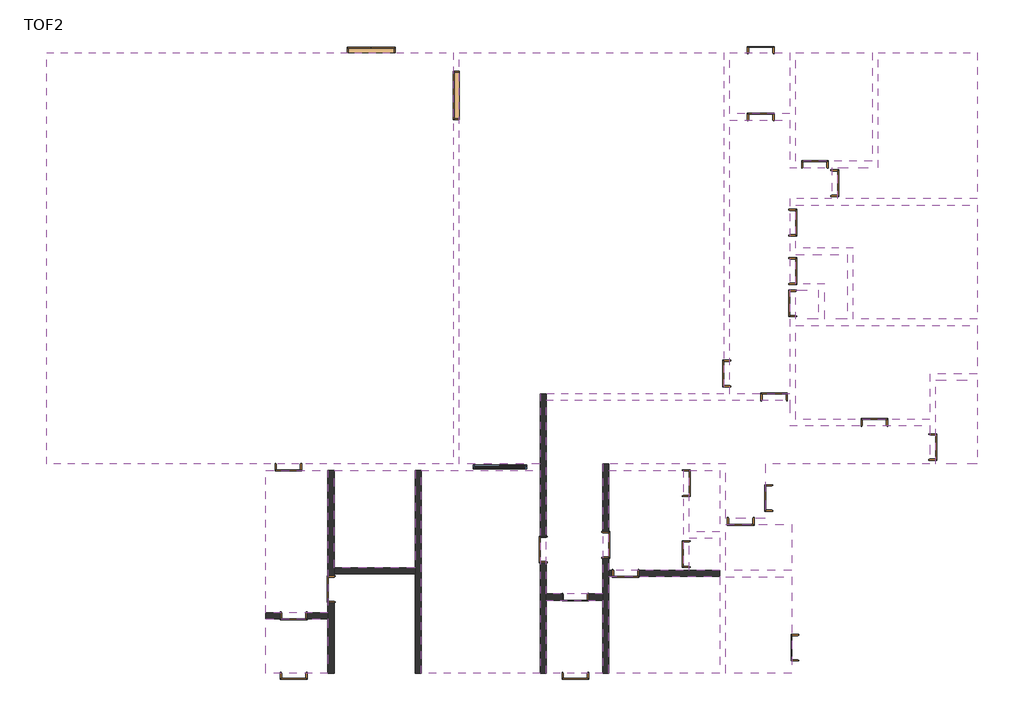
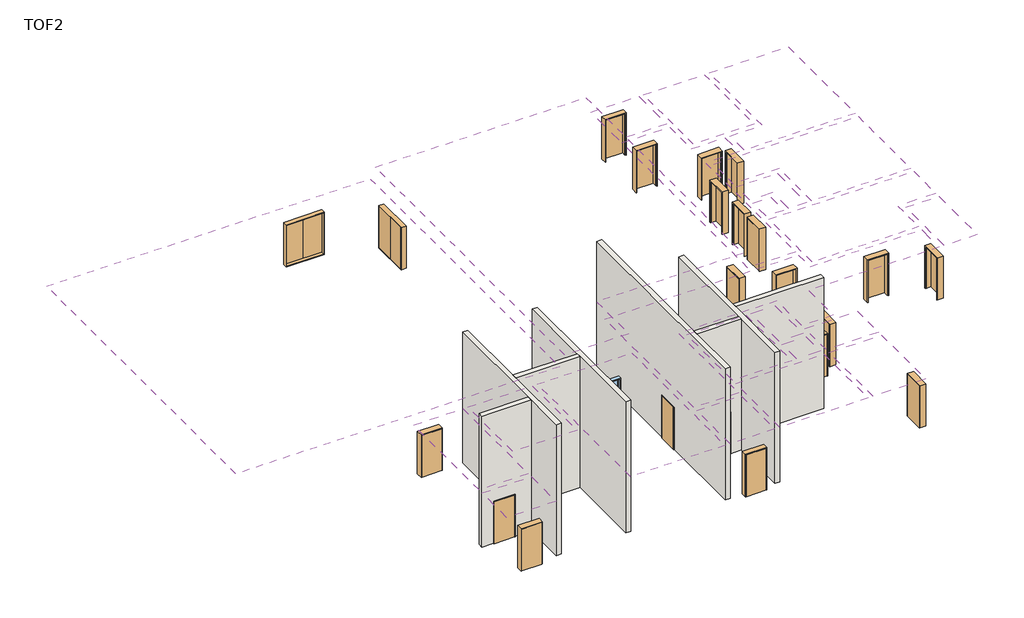
# One storey: 27 doors, 23 coverings, 8 walls, 1 window.
# Revit data of these elements (continued)
# Type "Sliding Window : H_WD_AR_B11_Sliding_Steel Window_DG_W2000xH1000" (continued)
#   Wall Closure = (empty or 0)
# Element 1 (IfcCovering, "H_CE_AR_B09_Acoustic Ceiling_T Bar_600x600x9T")
#   Height Offset From Level = 3000 mm
#   Phase Created = New Construction
# Element 2 (IfcCovering, "H_CE_AR_B09_Acoustic Ceiling_T Bar_600x600x9T")
#   Height Offset From Level = 3500 mm
#   Phase Created = New Construction
# Elements 3, 4, 5, 6, 7, 8, 9, 10, 11, 12, 13, 14, 15, 16, 17, 18, 19, 20, 21, 22, 23 (IfcCovering, "H_CE_AR_B09_Acoustic Ceiling_T Bar_600x600x9T")
#   Height Offset From Level = 2700 mm
#   Phase Created = New Construction
# Elements 24, 25 (IfcDoor, "Double Door_Steel : H_DR_AR_B12_Double Door_Steel_W2000xH2100")
#   H_Door Style Name = "Steel Door_Double"
#   H_Door_Frame = "Steel"
#   H_Door_Leaf = "Steel"
#   H_Door_Vision = "N.A"
#   H_Door_Panic = "N.A"
#   H_Door_Style Remark = ""
#   H_Door_Fire Rating = "NA/0.5/1.0\n/1.5/2.0"
#   H_Door Style No = DD11
#   Phase Created = New Construction
# Elements 26, 27, 28, 29, 30, 31, 32, 33, 34, 35, 36, 37, 38, 39, 40, 41, 42, 43, 44, 45, 46, 47, 48, 49, 50 (IfcDoor, "Single Door_Steel : H_DR_AR_B12_Single Door_Steel_W1000xH2100")
#   H_Door Style Name = "Steel Door_Single"
#   H_Door_Frame = "Steel"
#   H_Door_Leaf = "Steel"
#   H_Door_Vision = "N.A"
#   H_Door_Panic = "N.A"
#   H_Door_Style Remark = "Steel Door w/ Steel Frame"
#   H_Door_Fire Rating = "NA/0.5/1.0\n/1.5/2.0"
#   H_Door Style No = SD11
#   Phase Created = New Construction
# Elements 51, 52, 53, 54, 55, 56, 57, 58 (IfcWall, "H_WA_AR_B02_Int Wall_Block T200")
#   H_Wall Style Name = "Block Wall"
#   H_Wall-Base Material-1 = "Concrete Block"
#   H_Wall-Base Material-2 = ""
#   H_Wall_Finish-In = "Acrylic Emulsion Paint on Cement Plaster"
#   H_Wall_Base Material-3 = ""
#   H_Wall_Finish-Ex = "Acrylic Emulsion Paint on Cement Plaster"
#   H_Wall_Style Remark = "WM : Reinforced Concrete Block\n     50mm<THK≤100mm / 100mm<THK≤200mm / 200mm<THK"
#   Top Offset = 0 mm
#   Base Offset = 0 mm
#   wall height = 6500 mm
#   H_Wall Style No = IW21
#   Phase Created = New Construction
#   Base Constraint = TOF2
#   Top Constraint = TOC
#   Materials on its faces: "Default Wall"
# Element 59 (IfcWindow, "Sliding Window : H_WD_AR_B11_Sliding_Steel Window_DG_W2000xH1000")
#   Mark = "FRW-01"
#   H_Window Style Name = "Steel Window_DG_Comb"
#   H_Window_Glass = "Double Glazing"
#   H_Window_Frame = "Steel"
#   H_Window_Fire Rating = "NA/0.5/1.0"
#   H_Window_Style Remark = ""
#   H_Window Style No = WN42
#   Phase Created = New Construction
# Materials
#   "Default Wall": class "Miscellaneous", colour RGB 80 80 80, transparency 0
# Room at (8960, 18159.521) mm, phase "New Construction", upper level "TOC", upper offset 2000 mm, lower offset -2000 mm
#   Comments = ""
#   Number = "101"
#   Name = "MECHANICAL ROOM"
#   H_Floor Finish Style Name = "Non-Slip Epoxy Paint"
#   H_Floor Base Material = "Concrete Slab / Steel Trowel Finish"
#   H_Wall-Base Material-1 = "Masonry Wall"
#   H_Skirt Finish Style Name = "Epoxy Paint"
#   H_Wall-Base Material-2 = ""
#   H_Wall-Base Material-3 = "Plastering"
#   H_Floor-Base Material-1 = "Concrete Slab"
#   H_Floor-Base Material-2 = "Steel Trowel Finish"
#   H_Floor-Base Material-3 = ""
#   H_Floor-Base Material-4 = ""
#   H_Floor-Base Material-5 = ""
#   H_Floor Finish-1 = "Epoxy Paint"
#   H_Floor Finish-2 = ""
#   H_Floor Finish Remark = "*WM 기준 확인 필요 Epoxy Paint \n(용제형, 0.1mm 이하) : epoxy resin + polyamine hardener(경화제)"
#   H_Skirt Base Material = "Same as Wall"
#   H_Skirt-Base Material-1 = ""
#   H_Skirt-Base Material-2 = ""
#   H_Skirt-Base Material-3 = ""
#   H_Skirt-Base Material-4 = ""
#   H_Skirt-Base Material-5 = ""
#   H_Skirt Finish-1 = "Epoxy Paint"
#   H_Skirt Finish-2 = ""
#   H_Skirt Finish Remark = "SACE"
#   H_Wall Finish Style Name = "Acrylic Emulsion Paint"
#   H_Wall Base Material = "Masonry Wall / Cement Plaster"
#   H_Wall-Base Material-4 = ""
#   H_Wall-Base Material-5 = ""
#   H_Wall Finish-1 = "Acrylic Emulsion Paint"
#   H_Wall Finish-2 = ""
#   H_Wall Finish Remark = "T13 Plaster"
#   H_Ceiling Finish Style Name = "Acrylic Emulsion Paint"
#   H_Ceiling Base Material = "Concrete Slab / Fair Faced Concrete"
#   H_Ceiling-Base Material-1 = "(Concrete Slab)"
#   H_Ceiling-Base Material-2 = ""
#   H_Ceiling-Base Material-3 = ""
#   H_Ceiling-Base Material-4 = ""
#   H_Ceiling-Base Material-5 = ""
#   H_Ceiling Finish-1 = "Acrylic Emulsion Paint"
#   H_Ceiling Finish-2 = ""
#   H_Ceiling Finish Remark = "SACE"
#   Floor Finish Style No = F06A
#   Skirt Finish Style No = B03
#   Wall Finish Style No = W01B
#   Ceiling Finish Style No = C01
# Room at (8960, 6314.521) mm, phase "New Construction", upper level "TOC", upper offset 2000 mm, lower offset -2000 mm
#   Comments = ""
#   Number = "112"
#   Name = "ELECTRICAL ROOM(SS08)"
#   H_Floor Finish Style Name = "Non-Slip Epoxy Paint"
#   H_Floor Base Material = "Concrete Slab / Screed"
#   H_Wall-Base Material-1 = "Masonry Wall"
#   H_Skirt Finish Style Name = "Epoxy Paint"
#   H_Wall-Base Material-2 = ""
#   H_Wall-Base Material-3 = "Plastering"
#   H_Floor-Base Material-1 = "Concrete Slab"
#   H_Floor-Base Material-2 = ""
#   H_Floor-Base Material-3 = "Screed"
#   H_Floor-Base Material-4 = ""
#   H_Floor-Base Material-5 = ""
#   H_Floor Finish-1 = "Epoxy Paint"
#   H_Floor Finish-2 = ""
#   H_Floor Finish Remark = "*WM 기준 확인 필요 Epoxy Paint \n(용제형, 0.1mm 이하) : epoxy resin + polyamine hardener(경화제)"
#   H_Skirt Base Material = "Same as Wall"
#   H_Skirt-Base Material-1 = ""
#   H_Skirt-Base Material-2 = ""
#   H_Skirt-Base Material-3 = ""
#   H_Skirt-Base Material-4 = ""
#   H_Skirt-Base Material-5 = ""
#   H_Skirt Finish-1 = "Epoxy Paint"
#   H_Skirt Finish-2 = ""
#   H_Skirt Finish Remark = "SACE"
#   H_Wall Finish Style Name = "Acrylic Emulsion Paint"
#   H_Wall Base Material = "Masonry Wall / Cement Plaster"
#   H_Wall-Base Material-4 = ""
#   H_Wall-Base Material-5 = ""
#   H_Wall Finish-1 = "Acrylic Emulsion Paint"
#   H_Wall Finish-2 = ""
#   H_Wall Finish Remark = "T13 Plaster"
#   H_Ceiling Finish Style Name = "Acrylic Emulsion Paint"
#   H_Ceiling Base Material = "Concrete Slab / Fair Faced Concrete"
#   H_Ceiling-Base Material-1 = "(Concrete Slab)"
#   H_Ceiling-Base Material-2 = ""
#   H_Ceiling-Base Material-3 = ""
#   H_Ceiling-Base Material-4 = ""
#   H_Ceiling-Base Material-5 = ""
#   H_Ceiling Finish-1 = "Acrylic Emulsion Paint"
#   H_Ceiling Finish-2 = ""
#   H_Ceiling Finish Remark = "SACE"
#   Floor Finish Style No = F06B
#   Skirt Finish Style No = B03
#   Wall Finish Style No = W01B
#   Ceiling Finish Style No = C01
# Room at (25745, 16214.521) mm, phase "New Construction", upper level "TOC", upper offset 2000 mm, lower offset -2000 mm
#   Comments = ""
#   Number = "102"
#   Name = "RACK ROOM"
#   H_Floor Finish Style Name = "Anti-Dust Epoxy Paint / Anti-Static Vinyl Tile on Raised Floor"
#   H_Floor Base Material = "Concrete Slab / Steel Trowel Finish"
#   H_Wall-Base Material-1 = "Masonry Wall"
#   H_Skirt Finish Style Name = "Coved Vinyl Tile"
#   H_Wall-Base Material-2 = ""
#   H_Wall-Base Material-3 = "Plastering"
#   H_Floor-Base Material-1 = "Concrete Slab"
#   H_Floor-Base Material-2 = "Steel Trowel Finish"
#   H_Floor-Base Material-3 = ""
#   H_Floor-Base Material-4 = ""
#   H_Floor-Base Material-5 = "Raised Floor_Anti-Static Vinyl Tile"
#   H_Floor Finish-1 = "Anti-Dust Paint"
#   H_Floor Finish-2 = "Raised Floor_Anti-Static Vinyl Tile"
#   H_Floor Finish Remark = "600x600, H=1000"
#   H_Skirt Base Material = "Same as Wall"
#   H_Skirt-Base Material-1 = ""
#   H_Skirt-Base Material-2 = ""
#   H_Skirt-Base Material-3 = ""
#   H_Skirt-Base Material-4 = ""
#   H_Skirt-Base Material-5 = ""
#   H_Skirt Finish-1 = "Vinyl Tile"
#   H_Skirt Finish-2 = ""
#   H_Skirt Finish Remark = "Vinyl Tile = PVC Tile (polyvinyl chloride)"
#   H_Wall Finish Style Name = "Acrylic Emulsion Paint"
#   H_Wall Base Material = "Masonry Wall / Cement Plaster"
#   H_Wall-Base Material-4 = ""
#   H_Wall-Base Material-5 = ""
#   H_Wall Finish-1 = "Acrylic Emulsion Paint"
#   H_Wall Finish-2 = ""
#   H_Wall Finish Remark = "T13 Plaster"
#   H_Ceiling Finish Style Name = "Suspended Acoustic Tiled Ceiling (M-Bar)"
#   H_Ceiling Base Material = "Concrete Slab / Fair Faced Concrete"
#   H_Ceiling-Base Material-1 = "(Concrete Slab)"
#   H_Ceiling-Base Material-2 = "(Fair Faced Concrete)"
#   H_Ceiling-Base Material-3 = ""
#   H_Ceiling-Base Material-4 = ""
#   H_Ceiling-Base Material-5 = "Acoustic Tiled Ceiling System (M-Bar)"
#   H_Ceiling Finish-1 = "Acoustic Tiled Ceiling System (M-Bar)"
#   H_Ceiling Finish-2 = ""
#   H_Ceiling Finish Remark = ""
#   Floor Finish Style No = F91
#   Skirt Finish Style No = B35
#   Wall Finish Style No = W01B
#   Ceiling Finish Style No = C95A
# Room at (22095, 4359.521) mm, phase "New Construction", upper level "TOC", upper offset 2000 mm, lower offset -2000 mm
#   Comments = ""
#   Number = "114"
#   Name = "BATTERY ROOM"
#   H_Floor Finish Style Name = "Acid Resistant Ceramic Tile"
#   H_Floor Base Material = "Concrete Slab / Steel Trowel Finish"
#   H_Wall-Base Material-1 = "Masonry Wall"
#   H_Skirt Finish Style Name = "Coved Vinyl Tile"
#   H_Wall-Base Material-2 = ""
#   H_Wall-Base Material-3 = "Plastering"
#   H_Floor-Base Material-1 = "Concrete Slab"
#   H_Floor-Base Material-2 = "Steel Trowel Finish"
#   H_Floor-Base Material-3 = ""
#   H_Floor-Base Material-4 = ""
#   H_Floor-Base Material-5 = "Acid/Alkaline Resistant Tile"
#   H_Floor Finish-1 = "Acid/Alkaline Resistant Tile"
#   H_Floor Finish-2 = ""
#   H_Floor Finish Remark = "*WM : Bonding용 Mortar은 Tile에 포함\n*Slope 용 Screed만 별도 구분 (Concrete 바닥 단차 발생하는 경우 Only)"
#   H_Skirt Base Material = "Same as Wall"
#   H_Skirt-Base Material-1 = ""
#   H_Skirt-Base Material-2 = ""
#   H_Skirt-Base Material-3 = ""
#   H_Skirt-Base Material-4 = ""
#   H_Skirt-Base Material-5 = ""
#   H_Skirt Finish-1 = "Vinyl Tile"
#   H_Skirt Finish-2 = ""
#   H_Skirt Finish Remark = "Vinyl Tile = PVC Tile (polyvinyl chloride)"
#   H_Wall Finish Style Name = "Acid Resistant Paint"
#   H_Wall Base Material = "Masonry Wall / Cement Plaster"
#   H_Wall-Base Material-4 = ""
#   H_Wall-Base Material-5 = ""
#   H_Wall Finish-1 = "Acid/Alkaline Resistant Paint"
#   H_Wall Finish-2 = ""
#   H_Wall Finish Remark = "T13 Plaster"
#   H_Ceiling Finish Style Name = "Acrylic Emulsion Paint"
#   H_Ceiling Base Material = "Concrete Slab / Fair Faced Concrete"
#   H_Ceiling-Base Material-1 = "(Concrete Slab)"
#   H_Ceiling-Base Material-2 = ""
#   H_Ceiling-Base Material-3 = ""
#   H_Ceiling-Base Material-4 = ""
#   H_Ceiling-Base Material-5 = ""
#   H_Ceiling Finish-1 = "Acrylic Emulsion Paint"
#   H_Ceiling Finish-2 = ""
#   H_Ceiling Finish Remark = "SACE"
#   Floor Finish Style No = F32A
#   Skirt Finish Style No = B35
#   Wall Finish Style No = W04B
#   Ceiling Finish Style No = C01
# Room at (34300, 4359.521) mm, phase "New Construction", upper level "TOC", upper offset 2000 mm, lower offset -2000 mm
#   Comments = ""
#   Number = "118"
#   Name = "DRIVERS LOUNGE"
#   H_Floor Finish Style Name = "Vinyl Tile"
#   H_Floor Base Material = "Concrete Slab / Steel Trowel Finish"
#   H_Wall-Base Material-1 = "Masonry Wall"
#   H_Skirt Finish Style Name = "Coved Vinyl Tile"
#   H_Wall-Base Material-2 = ""
#   H_Wall-Base Material-3 = "Plastering"
#   H_Floor-Base Material-1 = "Concrete Slab"
#   H_Floor-Base Material-2 = "Steel Trowel Finish"
#   H_Floor-Base Material-3 = ""
#   H_Floor-Base Material-4 = ""
#   H_Floor-Base Material-5 = "Vinyl Tile"
#   H_Floor Finish-1 = "Vinyl Tile"
#   H_Floor Finish-2 = ""
#   H_Floor Finish Remark = ""
#   H_Skirt Base Material = "Same as Wall"
#   H_Skirt-Base Material-1 = ""
#   H_Skirt-Base Material-2 = ""
#   H_Skirt-Base Material-3 = ""
#   H_Skirt-Base Material-4 = ""
#   H_Skirt-Base Material-5 = ""
#   H_Skirt Finish-1 = "Vinyl Tile"
#   H_Skirt Finish-2 = ""
#   H_Skirt Finish Remark = "Vinyl Tile = PVC Tile (polyvinyl chloride)"
#   H_Wall Finish Style Name = "Acrylic Emulsion Paint"
#   H_Wall Base Material = "Masonry Wall / Cement Plaster"
#   H_Wall-Base Material-4 = ""
#   H_Wall-Base Material-5 = ""
#   H_Wall Finish-1 = "Acrylic Emulsion Paint"
#   H_Wall Finish-2 = ""
#   H_Wall Finish Remark = "T13 Plaster"
#   H_Ceiling Finish Style Name = "Suspended Acoustic Tiled Ceiling (M-Bar)"
#   H_Ceiling Base Material = "Concrete Slab / Fair Faced Concrete"
#   H_Ceiling-Base Material-1 = "(Concrete Slab)"
#   H_Ceiling-Base Material-2 = "(Fair Faced Concrete)"
#   H_Ceiling-Base Material-3 = ""
#   H_Ceiling-Base Material-4 = ""
#   H_Ceiling-Base Material-5 = "Acoustic Tiled Ceiling System (M-Bar)"
#   H_Ceiling Finish-1 = "Acoustic Tiled Ceiling System (M-Bar)"
#   H_Ceiling Finish-2 = ""
#   H_Ceiling Finish Remark = ""
#   Floor Finish Style No = F34A
#   Skirt Finish Style No = B35
#   Wall Finish Style No = W01B
#   Ceiling Finish Style No = C95A
# Room at (38475, 15984.521) mm, phase "New Construction", upper level "TOC", upper offset 2000 mm, lower offset -2000 mm
#   Comments = ""
#   Number = "103"
#   Name = "CONTROL ROOM"
#   H_Floor Finish Style Name = "Anti-Dust Epoxy Paint / Anti-Static Vinyl Tile on Raised Floor"
#   H_Floor Base Material = "Concrete Slab / Steel Trowel Finish"
#   H_Wall-Base Material-1 = "Masonry Wall"
#   H_Skirt Finish Style Name = "Coved Vinyl Tile"
#   H_Wall-Base Material-2 = ""
#   H_Wall-Base Material-3 = "Plastering"
#   H_Floor-Base Material-1 = "Concrete Slab"
#   H_Floor-Base Material-2 = "Steel Trowel Finish"
#   H_Floor-Base Material-3 = ""
#   H_Floor-Base Material-4 = ""
#   H_Floor-Base Material-5 = "Raised Floor_Anti-Static Vinyl Tile"
#   H_Floor Finish-1 = "Anti-Dust Paint"
#   H_Floor Finish-2 = "Raised Floor_Anti-Static Vinyl Tile"
#   H_Floor Finish Remark = "600x600, H=1000"
#   H_Skirt Base Material = "Same as Wall"
#   H_Skirt-Base Material-1 = ""
#   H_Skirt-Base Material-2 = ""
#   H_Skirt-Base Material-3 = ""
#   H_Skirt-Base Material-4 = ""
#   H_Skirt-Base Material-5 = ""
#   H_Skirt Finish-1 = "Vinyl Tile"
#   H_Skirt Finish-2 = ""
#   H_Skirt Finish Remark = "Vinyl Tile = PVC Tile (polyvinyl chloride)"
#   H_Wall Finish Style Name = "Acrylic Emulsion Paint"
#   H_Wall Base Material = "Masonry Wall / Cement Plaster"
#   H_Wall-Base Material-4 = ""
#   H_Wall-Base Material-5 = ""
#   H_Wall Finish-1 = "Acrylic Emulsion Paint"
#   H_Wall Finish-2 = ""
#   H_Wall Finish Remark = "T13 Plaster"
#   H_Ceiling Finish Style Name = "Suspended Acoustic Tiled Ceiling (M-Bar)"
#   H_Ceiling Base Material = "Concrete Slab / Fair Faced Concrete"
#   H_Ceiling-Base Material-1 = "(Concrete Slab)"
#   H_Ceiling-Base Material-2 = "(Fair Faced Concrete)"
#   H_Ceiling-Base Material-3 = ""
#   H_Ceiling-Base Material-4 = ""
#   H_Ceiling-Base Material-5 = "Acoustic Tiled Ceiling System (M-Bar)"
#   H_Ceiling Finish-1 = "Acoustic Tiled Ceiling System (M-Bar)"
#   H_Ceiling Finish-2 = ""
#   H_Ceiling Finish Remark = ""
#   Floor Finish Style No = F91
#   Skirt Finish Style No = B35
#   Wall Finish Style No = W01B
#   Ceiling Finish Style No = C95A
# Room at (41230, 2411.673) mm, phase "New Construction", upper level "TOC", upper offset 2000 mm, lower offset -2000 mm
#   Comments = ""
#   Number = "122"
#   Name = "TOILETS"
#   H_Floor Finish Style Name = "Non-Slip Unglazed Ceramic Tile"
#   H_Floor Base Material = "Concrete Slab / Screed / Liquid Waterproofing"
#   H_Wall-Base Material-1 = "Masonry Wall"
#   H_Skirt Finish Style Name = "Coved Ceramic Tile"
#   H_Wall-Base Material-2 = ""
#   H_Wall-Base Material-3 = ""
#   H_Floor-Base Material-1 = "Concrete Slab"
#   H_Floor-Base Material-2 = ""
#   H_Floor-Base Material-3 = "Screed"
#   H_Floor-Base Material-4 = "Liquid Waterproofing"
#   H_Floor-Base Material-5 = "Ceramic Tile"
#   H_Floor Finish-1 = "Ceramic Tile"
#   H_Floor Finish-2 = ""
#   H_Floor Finish Remark = ""
#   H_Skirt Base Material = "Same as Wall"
#   H_Skirt-Base Material-1 = ""
#   H_Skirt-Base Material-2 = ""
#   H_Skirt-Base Material-3 = ""
#   H_Skirt-Base Material-4 = ""
#   H_Skirt-Base Material-5 = ""
#   H_Skirt Finish-1 = "Glazed Ceramic Tile"
#   H_Skirt Finish-2 = ""
#   H_Skirt Finish Remark = ""
#   H_Wall Finish Style Name = "Glazed Ceramic Tile (≤C.H+100) / No Paint (>C.H+100)"
#   H_Wall Base Material = "Masonry Wall / Liquid Waterproofing"
#   H_Wall-Base Material-4 = "Liquid Waterproofing"
#   H_Wall-Base Material-5 = "Glazed Ceramic Tile"
#   H_Wall Finish-1 = "Glazed Ceramic Tile"
#   H_Wall Finish-2 = ""
#   H_Wall Finish Remark = "Below Suspended Ceiling\nGlazed Ceramic Tile(≤C.H+100) + Liquid Waterproofing / No Paint (>C.H+100)"
#   H_Ceiling Finish Style Name = "Suspended Moisture Resistant Tiled Ceiling (M-Bar)"
#   H_Ceiling Base Material = "Concrete Slab / Fair Faced Concrete"
#   H_Ceiling-Base Material-1 = "(Concrete Slab)"
#   H_Ceiling-Base Material-2 = "(Fair Faced Concrete)"
#   H_Ceiling-Base Material-3 = ""
#   H_Ceiling-Base Material-4 = ""
#   H_Ceiling-Base Material-5 = "Moisture Resistant Tiled Ceiling System (M-Bar)"
#   H_Ceiling Finish-1 = "Moisture Resistant Tiled Ceiling System (M-Bar)"
#   H_Ceiling Finish-2 = ""
#   H_Ceiling Finish Remark = ""
#   Floor Finish Style No = F31B
#   Skirt Finish Style No = B32
#   Wall Finish Style No = W32B
#   Ceiling Finish Style No = C96A
# Room at (49122.5, 4434.521) mm, phase "New Construction", upper level "TOC", upper offset 2000 mm, lower offset -2000 mm
#   Comments = ""
#   Number = "125"
#   Name = "MAINTENANCE WORKSHOP"
#   H_Floor Finish Style Name = "Non-Slip Epoxy Paint"
#   H_Floor Base Material = "Concrete Slab / Steel Trowel Finish"
#   H_Wall-Base Material-1 = "Masonry Wall"
#   H_Skirt Finish Style Name = "Epoxy Paint"
#   H_Wall-Base Material-2 = ""
#   H_Wall-Base Material-3 = "Plastering"
#   H_Floor-Base Material-1 = "Concrete Slab"
#   H_Floor-Base Material-2 = "Steel Trowel Finish"
#   H_Floor-Base Material-3 = ""
#   H_Floor-Base Material-4 = ""
#   H_Floor-Base Material-5 = ""
#   H_Floor Finish-1 = "Epoxy Paint"
#   H_Floor Finish-2 = ""
#   H_Floor Finish Remark = "*WM 기준 확인 필요 Epoxy Paint \n(용제형, 0.1mm 이하) : epoxy resin + polyamine hardener(경화제)"
#   H_Skirt Base Material = "Same as Wall"
#   H_Skirt-Base Material-1 = ""
#   H_Skirt-Base Material-2 = ""
#   H_Skirt-Base Material-3 = ""
#   H_Skirt-Base Material-4 = ""
#   H_Skirt-Base Material-5 = ""
#   H_Skirt Finish-1 = "Epoxy Paint"
#   H_Skirt Finish-2 = ""
#   H_Skirt Finish Remark = "SACE"
#   H_Wall Finish Style Name = "Acrylic Emulsion Paint"
#   H_Wall Base Material = "Masonry Wall / Cement Plaster"
#   H_Wall-Base Material-4 = ""
#   H_Wall-Base Material-5 = ""
#   H_Wall Finish-1 = "Acrylic Emulsion Paint"
#   H_Wall Finish-2 = ""
#   H_Wall Finish Remark = "T13 Plaster"
#   H_Ceiling Finish Style Name = "Acrylic Emulsion Paint"
#   H_Ceiling Base Material = "Concrete Slab / Fair Faced Concrete"
#   H_Ceiling-Base Material-1 = "(Concrete Slab)"
#   H_Ceiling-Base Material-2 = ""
#   H_Ceiling-Base Material-3 = ""
#   H_Ceiling-Base Material-4 = ""
#   H_Ceiling-Base Material-5 = ""
#   H_Ceiling Finish-1 = "Acrylic Emulsion Paint"
#   H_Ceiling Finish-2 = ""
#   H_Ceiling Finish Remark = "SACE"
#   Floor Finish Style No = F06A
#   Skirt Finish Style No = B03
#   Wall Finish Style No = W01B
#   Ceiling Finish Style No = C01
# Room at (40475, 6276.673) mm, phase "New Construction", upper level "TOC", upper offset 2000 mm, lower offset -2000 mm
#   Comments = ""
#   Number = "121"
#   Name = "LOCKER"
#   H_Floor Finish Style Name = "Non-Slip Unglazed Ceramic Tile"
#   H_Floor Base Material = "Concrete Slab / Steel Trowel Finish"
#   H_Wall-Base Material-1 = "Masonry Wall"
#   H_Skirt Finish Style Name = "Coved Ceramic Tile"
#   H_Wall-Base Material-2 = ""
#   H_Wall-Base Material-3 = ""
#   H_Floor-Base Material-1 = "Concrete Slab"
#   H_Floor-Base Material-2 = "Steel Trowel Finish"
#   H_Floor-Base Material-3 = ""
#   H_Floor-Base Material-4 = ""
#   H_Floor-Base Material-5 = "Ceramic Tile"
#   H_Floor Finish-1 = "Ceramic Tile"
#   H_Floor Finish-2 = ""
#   H_Floor Finish Remark = "*WM : Bonding용 Mortar은 Tile에 포함\n*Slope 용 Screed만 별도 구분 (Concrete 바닥 단차 발생하는 경우 Only)"
#   H_Skirt Base Material = "Same as Wall"
#   H_Skirt-Base Material-1 = ""
#   H_Skirt-Base Material-2 = ""
#   H_Skirt-Base Material-3 = ""
#   H_Skirt-Base Material-4 = ""
#   H_Skirt-Base Material-5 = ""
#   H_Skirt Finish-1 = "Glazed Ceramic Tile"
#   H_Skirt Finish-2 = ""
#   H_Skirt Finish Remark = ""
#   H_Wall Finish Style Name = "Glazed Ceramic Tile (≤C.H+100) / No Paint (>C.H+100)"
#   H_Wall Base Material = "Masonry Wall / Liquid Waterproofing"
#   H_Wall-Base Material-4 = "Liquid Waterproofing"
#   H_Wall-Base Material-5 = "Glazed Ceramic Tile"
#   H_Wall Finish-1 = "Glazed Ceramic Tile"
#   H_Wall Finish-2 = ""
#   H_Wall Finish Remark = "Below Suspended Ceiling\nGlazed Ceramic Tile(≤C.H+100) + Liquid Waterproofing / No Paint (>C.H+100)"
#   H_Ceiling Finish Style Name = "Suspended Moisture Resistant Tiled Ceiling (M-Bar)"
#   H_Ceiling Base Material = "Concrete Slab / Fair Faced Concrete"
#   H_Ceiling-Base Material-1 = "(Concrete Slab)"
#   H_Ceiling-Base Material-2 = "(Fair Faced Concrete)"
#   H_Ceiling-Base Material-3 = ""
#   H_Ceiling-Base Material-4 = ""
#   H_Ceiling-Base Material-5 = "Moisture Resistant Tiled Ceiling System (M-Bar)"
#   H_Ceiling Finish-1 = "Moisture Resistant Tiled Ceiling System (M-Bar)"
#   H_Ceiling Finish-2 = ""
#   H_Ceiling Finish Remark = ""
#   Floor Finish Style No = F31A
#   Skirt Finish Style No = B32
#   Wall Finish Style No = W32B
#   Ceiling Finish Style No = C96A
# Room at (42700, 7069.521) mm, phase "New Construction", upper level "TOC", upper offset 2000 mm, lower offset -2000 mm
#   Comments = ""
#   Number = "127"
#   Name = "SHOWER ROOM"
#   H_Floor Finish Style Name = "Non-Slip Unglazed Ceramic Tile"
#   H_Floor Base Material = "Concrete Slab / Screed / Liquid Waterproofing"
#   H_Wall-Base Material-1 = "Concrete Wall"
#   H_Skirt Finish Style Name = "Epoxy Paint"
#   H_Wall-Base Material-2 = ""
#   H_Wall-Base Material-3 = ""
#   H_Floor-Base Material-1 = "Concrete Slab"
#   H_Floor-Base Material-2 = ""
#   H_Floor-Base Material-3 = "Screed"
#   H_Floor-Base Material-4 = "Liquid Waterproofing"
#   H_Floor-Base Material-5 = "Ceramic Tile"
#   H_Floor Finish-1 = "Ceramic Tile"
#   H_Floor Finish-2 = ""
#   H_Floor Finish Remark = ""
#   H_Skirt Base Material = "Same as Wall"
#   H_Skirt-Base Material-1 = ""
#   H_Skirt-Base Material-2 = ""
#   H_Skirt-Base Material-3 = ""
#   H_Skirt-Base Material-4 = ""
#   H_Skirt-Base Material-5 = ""
#   H_Skirt Finish-1 = "Epoxy Paint"
#   H_Skirt Finish-2 = ""
#   H_Skirt Finish Remark = "SACE"
#   H_Wall Finish Style Name = "Glazed Ceramic Tile (≤C.H+100) / No Paint (>C.H+100)"
#   H_Wall Base Material = "Concrete Wall"
#   H_Wall-Base Material-4 = "No Waterproofing"
#   H_Wall-Base Material-5 = "Glazed Ceramic Tile"
#   H_Wall Finish-1 = "Glazed Ceramic Tile"
#   H_Wall Finish-2 = ""
#   H_Wall Finish Remark = "Below Suspended Ceiling\nGlazed Ceramic Tile(≤C.H+100) / No Paint (>C.H+100)"
#   H_Ceiling Finish Style Name = "Suspended Moisture Resistant Tiled Ceiling (M-Bar)"
#   H_Ceiling Base Material = "Concrete Slab / Fair Faced Concrete"
#   H_Ceiling-Base Material-1 = "(Concrete Slab)"
#   H_Ceiling-Base Material-2 = "(Fair Faced Concrete)"
#   H_Ceiling-Base Material-3 = ""
#   H_Ceiling-Base Material-4 = ""
#   H_Ceiling-Base Material-5 = "Moisture Resistant Tiled Ceiling System (M-Bar)"
#   H_Ceiling Finish-1 = "Moisture Resistant Tiled Ceiling System (M-Bar)"
#   H_Ceiling Finish-2 = ""
#   H_Ceiling Finish Remark = ""
#   Floor Finish Style No = F31B
#   Skirt Finish Style No = B03
#   Wall Finish Style No = W32C
#   Ceiling Finish Style No = C96A
# Room at (42700, 5046.673) mm, phase "New Construction", upper level "TOC", upper offset 2000 mm, lower offset -2000 mm
#   Comments = ""
#   Number = "128"
#   Name = "EWH ROOM"
#   H_Floor Finish Style Name = "Non-Slip Unglazed Ceramic Tile"
#   H_Floor Base Material = "Concrete Slab / Steel Trowel Finish"
#   H_Wall-Base Material-1 = "Masonry Wall"
#   H_Skirt Finish Style Name = "Epoxy Paint"
#   H_Wall-Base Material-2 = ""
#   H_Wall-Base Material-3 = "Plastering"
#   H_Floor-Base Material-1 = "Concrete Slab"
#   H_Floor-Base Material-2 = "Steel Trowel Finish"
#   H_Floor-Base Material-3 = ""
#   H_Floor-Base Material-4 = ""
#   H_Floor-Base Material-5 = "Ceramic Tile"
#   H_Floor Finish-1 = "Ceramic Tile"
#   H_Floor Finish-2 = ""
#   H_Floor Finish Remark = "*WM : Bonding용 Mortar은 Tile에 포함\n*Slope 용 Screed만 별도 구분 (Concrete 바닥 단차 발생하는 경우 Only)"
#   H_Skirt Base Material = "Same as Wall"
#   H_Skirt-Base Material-1 = ""
#   H_Skirt-Base Material-2 = ""
#   H_Skirt-Base Material-3 = ""
#   H_Skirt-Base Material-4 = ""
#   H_Skirt-Base Material-5 = ""
#   H_Skirt Finish-1 = "Epoxy Paint"
#   H_Skirt Finish-2 = ""
#   H_Skirt Finish Remark = "SACE"
#   H_Wall Finish Style Name = "Acrylic Emulsion Paint"
#   H_Wall Base Material = "Masonry Wall / Cement Plaster"
#   H_Wall-Base Material-4 = ""
#   H_Wall-Base Material-5 = ""
#   H_Wall Finish-1 = "Acrylic Emulsion Paint"
#   H_Wall Finish-2 = ""
#   H_Wall Finish Remark = "T13 Plaster"
#   H_Ceiling Finish Style Name = "Suspended Acoustic Tiled Ceiling (M-Bar)"
#   H_Ceiling Base Material = "Concrete Slab / Fair Faced Concrete"
#   H_Ceiling-Base Material-1 = "(Concrete Slab)"
#   H_Ceiling-Base Material-2 = "(Fair Faced Concrete)"
#   H_Ceiling-Base Material-3 = ""
#   H_Ceiling-Base Material-4 = ""
#   H_Ceiling-Base Material-5 = "Acoustic Tiled Ceiling System (M-Bar)"
#   H_Ceiling Finish-1 = "Acoustic Tiled Ceiling System (M-Bar)"
#   H_Ceiling Finish-2 = ""
#   H_Ceiling Finish Remark = ""
#   Floor Finish Style No = F31A
#   Skirt Finish Style No = B03
#   Wall Finish Style No = W01B
#   Ceiling Finish Style No = C95A
# Room at (52040, 9944.521) mm, phase "New Construction", upper level "TOC", upper offset 2000 mm, lower offset -2000 mm
#   Comments = ""
#   Number = "110"
#   Name = "ABLUTIONS"
#   H_Floor Finish Style Name = "Non-Slip Unglazed Ceramic Tile"
#   H_Floor Base Material = "Concrete Slab / Screed / Liquid Waterproofing"
#   H_Wall-Base Material-1 = "Masonry Wall"
#   H_Skirt Finish Style Name = "Coved Ceramic Tile"
#   H_Wall-Base Material-2 = ""
#   H_Wall-Base Material-3 = ""
#   H_Floor-Base Material-1 = "Concrete Slab"
#   H_Floor-Base Material-2 = ""
#   H_Floor-Base Material-3 = "Screed"
#   H_Floor-Base Material-4 = "Liquid Waterproofing"
#   H_Floor-Base Material-5 = "Ceramic Tile"
#   H_Floor Finish-1 = "Ceramic Tile"
#   H_Floor Finish-2 = ""
#   H_Floor Finish Remark = ""
#   H_Skirt Base Material = "Same as Wall"
#   H_Skirt-Base Material-1 = ""
#   H_Skirt-Base Material-2 = ""
#   H_Skirt-Base Material-3 = ""
#   H_Skirt-Base Material-4 = ""
#   H_Skirt-Base Material-5 = ""
#   H_Skirt Finish-1 = "Glazed Ceramic Tile"
#   H_Skirt Finish-2 = ""
#   H_Skirt Finish Remark = ""
#   H_Wall Finish Style Name = "Glazed Ceramic Tile (≤C.H+100) / No Paint (>C.H+100)"
#   H_Wall Base Material = "Masonry Wall / Liquid Waterproofing"
#   H_Wall-Base Material-4 = "Liquid Waterproofing"
#   H_Wall-Base Material-5 = "Glazed Ceramic Tile"
#   H_Wall Finish-1 = "Glazed Ceramic Tile"
#   H_Wall Finish-2 = ""
#   H_Wall Finish Remark = "Below Suspended Ceiling\nGlazed Ceramic Tile(≤C.H+100) + Liquid Waterproofing / No Paint (>C.H+100)"
#   H_Ceiling Finish Style Name = "Suspended Moisture Resistant Tiled Ceiling (M-Bar)"
#   H_Ceiling Base Material = "Concrete Slab / Fair Faced Concrete"
#   H_Ceiling-Base Material-1 = "(Concrete Slab)"
#   H_Ceiling-Base Material-2 = "(Fair Faced Concrete)"
#   H_Ceiling-Base Material-3 = ""
#   H_Ceiling-Base Material-4 = ""
#   H_Ceiling-Base Material-5 = "Moisture Resistant Tiled Ceiling System (M-Bar)"
#   H_Ceiling Finish-1 = "Moisture Resistant Tiled Ceiling System (M-Bar)"
#   H_Ceiling Finish-2 = ""
#   H_Ceiling Finish Remark = ""
#   Floor Finish Style No = F31B
#   Skirt Finish Style No = B32
#   Wall Finish Style No = W32B
#   Ceiling Finish Style No = C96A
# Room at (50360, 21134.521) mm, phase "New Construction", upper level "TOC", upper offset 2000 mm, lower offset -2000 mm
#   Comments = ""
#   Number = "106"
#   Name = "SHIFT SUPERVISOR/DAY SUPERVISOR"
#   H_Floor Finish Style Name = "Vinyl Tile"
#   H_Floor Base Material = "Concrete Slab / Steel Trowel Finish"
#   H_Wall-Base Material-1 = "Masonry Wall"
#   H_Skirt Finish Style Name = "Coved Vinyl Tile"
#   H_Wall-Base Material-2 = ""
#   H_Wall-Base Material-3 = "Plastering"
#   H_Floor-Base Material-1 = "Concrete Slab"
#   H_Floor-Base Material-2 = "Steel Trowel Finish"
#   H_Floor-Base Material-3 = ""
#   H_Floor-Base Material-4 = ""
#   H_Floor-Base Material-5 = "Vinyl Tile"
#   H_Floor Finish-1 = "Vinyl Tile"
#   H_Floor Finish-2 = ""
#   H_Floor Finish Remark = ""
#   H_Skirt Base Material = "Same as Wall"
#   H_Skirt-Base Material-1 = ""
#   H_Skirt-Base Material-2 = ""
#   H_Skirt-Base Material-3 = ""
#   H_Skirt-Base Material-4 = ""
#   H_Skirt-Base Material-5 = ""
#   H_Skirt Finish-1 = "Vinyl Tile"
#   H_Skirt Finish-2 = ""
#   H_Skirt Finish Remark = "Vinyl Tile = PVC Tile (polyvinyl chloride)"
#   H_Wall Finish Style Name = "Acrylic Emulsion Paint"
#   H_Wall Base Material = "Masonry Wall / Cement Plaster"
#   H_Wall-Base Material-4 = ""
#   H_Wall-Base Material-5 = ""
#   H_Wall Finish-1 = "Acrylic Emulsion Paint"
#   H_Wall Finish-2 = ""
#   H_Wall Finish Remark = "T13 Plaster"
#   H_Ceiling Finish Style Name = "Suspended Acoustic Tiled Ceiling (M-Bar)"
#   H_Ceiling Base Material = "Concrete Slab / Fair Faced Concrete"
#   H_Ceiling-Base Material-1 = "(Concrete Slab)"
#   H_Ceiling-Base Material-2 = "(Fair Faced Concrete)"
#   H_Ceiling-Base Material-3 = ""
#   H_Ceiling-Base Material-4 = ""
#   H_Ceiling-Base Material-5 = "Acoustic Tiled Ceiling System (M-Bar)"
#   H_Ceiling Finish-1 = "Acoustic Tiled Ceiling System (M-Bar)"
#   H_Ceiling Finish-2 = ""
#   H_Ceiling Finish Remark = ""
#   Floor Finish Style No = F34A
#   Skirt Finish Style No = B35
#   Wall Finish Style No = W01B
#   Ceiling Finish Style No = C95A
# Room at (44725, 22722.021) mm, phase "New Construction", upper level "TOC", upper offset 2000 mm, lower offset -2000 mm
#   Comments = ""
#   Number = "104"
#   Name = "AIR LOCK"
#   H_Floor Finish Style Name = "Vinyl Tile"
#   H_Floor Base Material = "Concrete Slab / Steel Trowel Finish"
#   H_Wall-Base Material-1 = "Masonry Wall"
#   H_Skirt Finish Style Name = "Coved Vinyl Tile"
#   H_Wall-Base Material-2 = ""
#   H_Wall-Base Material-3 = "Plastering"
#   H_Floor-Base Material-1 = "Concrete Slab"
#   H_Floor-Base Material-2 = "Steel Trowel Finish"
#   H_Floor-Base Material-3 = ""
#   H_Floor-Base Material-4 = ""
#   H_Floor-Base Material-5 = "Vinyl Tile"
#   H_Floor Finish-1 = "Vinyl Tile"
#   H_Floor Finish-2 = ""
#   H_Floor Finish Remark = ""
#   H_Skirt Base Material = "Same as Wall"
#   H_Skirt-Base Material-1 = ""
#   H_Skirt-Base Material-2 = ""
#   H_Skirt-Base Material-3 = ""
#   H_Skirt-Base Material-4 = ""
#   H_Skirt-Base Material-5 = ""
#   H_Skirt Finish-1 = "Vinyl Tile"
#   H_Skirt Finish-2 = ""
#   H_Skirt Finish Remark = "Vinyl Tile = PVC Tile (polyvinyl chloride)"
#   H_Wall Finish Style Name = "Acrylic Emulsion Paint"
#   H_Wall Base Material = "Masonry Wall / Cement Plaster"
#   H_Wall-Base Material-4 = ""
#   H_Wall-Base Material-5 = ""
#   H_Wall Finish-1 = "Acrylic Emulsion Paint"
#   H_Wall Finish-2 = ""
#   H_Wall Finish Remark = "T13 Plaster"
#   H_Ceiling Finish Style Name = "Suspended Acoustic Tiled Ceiling (M-Bar)"
#   H_Ceiling Base Material = "Concrete Slab / Fair Faced Concrete"
#   H_Ceiling-Base Material-1 = "(Concrete Slab)"
#   H_Ceiling-Base Material-2 = "(Fair Faced Concrete)"
#   H_Ceiling-Base Material-3 = ""
#   H_Ceiling-Base Material-4 = ""
#   H_Ceiling-Base Material-5 = "Acoustic Tiled Ceiling System (M-Bar)"
#   H_Ceiling Finish-1 = "Acoustic Tiled Ceiling System (M-Bar)"
#   H_Ceiling Finish-2 = ""
#   H_Ceiling Finish Remark = ""
#   Floor Finish Style No = F34A
#   Skirt Finish Style No = B35
#   Wall Finish Style No = W01B
#   Ceiling Finish Style No = C95A
# Room at (45470, 16157.021) mm, phase "New Construction", upper level "TOC", upper offset 2000 mm, lower offset -2000 mm
#   Comments = ""
#   Number = "107"
#   Name = "CORRIDOR"
#   H_Floor Finish Style Name = "Vinyl Tile"
#   H_Floor Base Material = "Concrete Slab / Steel Trowel Finish"
#   H_Wall-Base Material-1 = "Masonry Wall"
#   H_Skirt Finish Style Name = "Coved Vinyl Tile"
#   H_Wall-Base Material-2 = ""
#   H_Wall-Base Material-3 = "Plastering"
#   H_Floor-Base Material-1 = "Concrete Slab"
#   H_Floor-Base Material-2 = "Steel Trowel Finish"
#   H_Floor-Base Material-3 = ""
#   H_Floor-Base Material-4 = ""
#   H_Floor-Base Material-5 = "Vinyl Tile"
#   H_Floor Finish-1 = "Vinyl Tile"
#   H_Floor Finish-2 = ""
#   H_Floor Finish Remark = ""
#   H_Skirt Base Material = "Same as Wall"
#   H_Skirt-Base Material-1 = ""
#   H_Skirt-Base Material-2 = ""
#   H_Skirt-Base Material-3 = ""
#   H_Skirt-Base Material-4 = ""
#   H_Skirt-Base Material-5 = ""
#   H_Skirt Finish-1 = "Vinyl Tile"
#   H_Skirt Finish-2 = ""
#   H_Skirt Finish Remark = "Vinyl Tile = PVC Tile (polyvinyl chloride)"
#   H_Wall Finish Style Name = "Acrylic Emulsion Paint"
#   H_Wall Base Material = "Masonry Wall / Cement Plaster"
#   H_Wall-Base Material-4 = ""
#   H_Wall-Base Material-5 = ""
#   H_Wall Finish-1 = "Acrylic Emulsion Paint"
#   H_Wall Finish-2 = ""
#   H_Wall Finish Remark = "T13 Plaster"
#   H_Ceiling Finish Style Name = "Suspended Acoustic Tiled Ceiling (M-Bar)"
#   H_Ceiling Base Material = "Concrete Slab / Fair Faced Concrete"
#   H_Ceiling-Base Material-1 = "(Concrete Slab)"
#   H_Ceiling-Base Material-2 = "(Fair Faced Concrete)"
#   H_Ceiling-Base Material-3 = ""
#   H_Ceiling-Base Material-4 = ""
#   H_Ceiling-Base Material-5 = "Acoustic Tiled Ceiling System (M-Bar)"
#   H_Ceiling Finish-1 = "Acoustic Tiled Ceiling System (M-Bar)"
#   H_Ceiling Finish-2 = ""
#   H_Ceiling Finish Remark = ""
#   Floor Finish Style No = F34A
#   Skirt Finish Style No = B35
#   Wall Finish Style No = W01B
#   Ceiling Finish Style No = C95A
# Room at (47500, 21684.521) mm, phase "New Construction", upper level "TOC", upper offset 2000 mm, lower offset -2000 mm
#   Comments = ""
#   Number = "105"
#   Name = "LIBRARY"
#   H_Floor Finish Style Name = "Vinyl Tile"
#   H_Floor Base Material = "Concrete Slab / Steel Trowel Finish"
#   H_Wall-Base Material-1 = "Masonry Wall"
#   H_Skirt Finish Style Name = "Coved Vinyl Tile"
#   H_Wall-Base Material-2 = ""
#   H_Wall-Base Material-3 = "Plastering"
#   H_Floor-Base Material-1 = "Concrete Slab"
#   H_Floor-Base Material-2 = "Steel Trowel Finish"
#   H_Floor-Base Material-3 = ""
#   H_Floor-Base Material-4 = ""
#   H_Floor-Base Material-5 = "Vinyl Tile"
#   H_Floor Finish-1 = "Vinyl Tile"
#   H_Floor Finish-2 = ""
#   H_Floor Finish Remark = ""
#   H_Skirt Base Material = "Same as Wall"
#   H_Skirt-Base Material-1 = ""
#   H_Skirt-Base Material-2 = ""
#   H_Skirt-Base Material-3 = ""
#   H_Skirt-Base Material-4 = ""
#   H_Skirt-Base Material-5 = ""
#   H_Skirt Finish-1 = "Vinyl Tile"
#   H_Skirt Finish-2 = ""
#   H_Skirt Finish Remark = "Vinyl Tile = PVC Tile (polyvinyl chloride)"
#   H_Wall Finish Style Name = "Acrylic Emulsion Paint"
#   H_Wall Base Material = "Masonry Wall / Cement Plaster"
#   H_Wall-Base Material-4 = ""
#   H_Wall-Base Material-5 = ""
#   H_Wall Finish-1 = "Acrylic Emulsion Paint"
#   H_Wall Finish-2 = ""
#   H_Wall Finish Remark = "T13 Plaster"
#   H_Ceiling Finish Style Name = "Suspended Acoustic Tiled Ceiling (M-Bar)"
#   H_Ceiling Base Material = "Concrete Slab / Fair Faced Concrete"
#   H_Ceiling-Base Material-1 = "(Concrete Slab)"
#   H_Ceiling-Base Material-2 = "(Fair Faced Concrete)"
#   H_Ceiling-Base Material-3 = ""
#   H_Ceiling-Base Material-4 = ""
#   H_Ceiling-Base Material-5 = "Acoustic Tiled Ceiling System (M-Bar)"
#   H_Ceiling Finish-1 = "Acoustic Tiled Ceiling System (M-Bar)"
#   H_Ceiling Finish-2 = ""
#   H_Ceiling Finish Remark = ""
#   Floor Finish Style No = F34A
#   Skirt Finish Style No = B35
#   Wall Finish Style No = W01B
#   Ceiling Finish Style No = C95A
# Room at (49385, 11844.521) mm, phase "New Construction", upper level "TOC", upper offset 2000 mm, lower offset -2000 mm
#   Comments = ""
#   Number = "111"
#   Name = "PRAYER ROOM"
#   H_Floor Finish Style Name = "Carpet"
#   H_Floor Base Material = "(기존 Floor Finish)"
#   H_Wall-Base Material-1 = "Masonry Wall"
#   H_Skirt Finish Style Name = "Coved Vinyl Tile"
#   H_Wall-Base Material-2 = ""
#   H_Wall-Base Material-3 = "Plastering"
#   H_Floor-Base Material-1 = "Carpet"
#   H_Floor-Base Material-2 = ""
#   H_Floor-Base Material-3 = ""
#   H_Floor-Base Material-4 = ""
#   H_Floor-Base Material-5 = ""
#   H_Floor Finish-1 = ""
#   H_Floor Finish-2 = ""
#   H_Floor Finish Remark = "* 기존 Floor Finsh 위에 Mat 의 설치면적 만큼 별도의 Family 적용"
#   H_Skirt Base Material = "Same as Wall"
#   H_Skirt-Base Material-1 = ""
#   H_Skirt-Base Material-2 = ""
#   H_Skirt-Base Material-3 = ""
#   H_Skirt-Base Material-4 = ""
#   H_Skirt-Base Material-5 = ""
#   H_Skirt Finish-1 = "Vinyl Tile"
#   H_Skirt Finish-2 = ""
#   H_Skirt Finish Remark = "Vinyl Tile = PVC Tile (polyvinyl chloride)"
#   H_Wall Finish Style Name = "Acrylic Emulsion Paint"
#   H_Wall Base Material = "Masonry Wall / Cement Plaster"
#   H_Wall-Base Material-4 = ""
#   H_Wall-Base Material-5 = ""
#   H_Wall Finish-1 = "Acrylic Emulsion Paint"
#   H_Wall Finish-2 = ""
#   H_Wall Finish Remark = "T13 Plaster"
#   H_Ceiling Finish Style Name = "Suspended Acoustic Tiled Ceiling (M-Bar)"
#   H_Ceiling Base Material = "Concrete Slab / Fair Faced Concrete"
#   H_Ceiling-Base Material-1 = "(Concrete Slab)"
#   H_Ceiling-Base Material-2 = "(Fair Faced Concrete)"
#   H_Ceiling-Base Material-3 = ""
#   H_Ceiling-Base Material-4 = ""
#   H_Ceiling-Base Material-5 = "Acoustic Tiled Ceiling System (M-Bar)"
#   H_Ceiling Finish-1 = "Acoustic Tiled Ceiling System (M-Bar)"
#   H_Ceiling Finish-2 = ""
#   H_Ceiling Finish Remark = ""
#   Floor Finish Style No = F71
#   Skirt Finish Style No = B35
#   Wall Finish Style No = W01B
#   Ceiling Finish Style No = C95A
# Room at (49615, 15969.521) mm, phase "New Construction", upper level "TOC", upper offset 2000 mm, lower offset -2000 mm
#   Comments = ""
#   Number = "108"
#   Name = "BREAK ROOM"
#   H_Floor Finish Style Name = "Vinyl Tile"
#   H_Floor Base Material = "Concrete Slab / Steel Trowel Finish"
#   H_Wall-Base Material-1 = "Masonry Wall"
#   H_Skirt Finish Style Name = "Coved Vinyl Tile"
#   H_Wall-Base Material-2 = ""
#   H_Wall-Base Material-3 = "Plastering"
#   H_Floor-Base Material-1 = "Concrete Slab"
#   H_Floor-Base Material-2 = "Steel Trowel Finish"
#   H_Floor-Base Material-3 = ""
#   H_Floor-Base Material-4 = ""
#   H_Floor-Base Material-5 = "Vinyl Tile"
#   H_Floor Finish-1 = "Vinyl Tile"
#   H_Floor Finish-2 = ""
#   H_Floor Finish Remark = ""
#   H_Skirt Base Material = "Same as Wall"
#   H_Skirt-Base Material-1 = ""
#   H_Skirt-Base Material-2 = ""
#   H_Skirt-Base Material-3 = ""
#   H_Skirt-Base Material-4 = ""
#   H_Skirt-Base Material-5 = ""
#   H_Skirt Finish-1 = "Vinyl Tile"
#   H_Skirt Finish-2 = ""
#   H_Skirt Finish Remark = "Vinyl Tile = PVC Tile (polyvinyl chloride)"
#   H_Wall Finish Style Name = "Acrylic Emulsion Paint"
#   H_Wall Base Material = "Masonry Wall / Cement Plaster"
#   H_Wall-Base Material-4 = ""
#   H_Wall-Base Material-5 = ""
#   H_Wall Finish-1 = "Acrylic Emulsion Paint"
#   H_Wall Finish-2 = ""
#   H_Wall Finish Remark = "T13 Plaster"
#   H_Ceiling Finish Style Name = "Suspended Moisture Resistant Tiled Ceiling (M-Bar)"
#   H_Ceiling Base Material = "Concrete Slab / Fair Faced Concrete"
#   H_Ceiling-Base Material-1 = "(Concrete Slab)"
#   H_Ceiling-Base Material-2 = "(Fair Faced Concrete)"
#   H_Ceiling-Base Material-3 = ""
#   H_Ceiling-Base Material-4 = ""
#   H_Ceiling-Base Material-5 = "Moisture Resistant Tiled Ceiling System (M-Bar)"
#   H_Ceiling Finish-1 = "Moisture Resistant Tiled Ceiling System (M-Bar)"
#   H_Ceiling Finish-2 = ""
#   H_Ceiling Finish Remark = ""
#   Floor Finish Style No = F34A
#   Skirt Finish Style No = B35
#   Wall Finish Style No = W01B
#   Ceiling Finish Style No = C96A
# Room at (47112.5, 15044.521) mm, phase "New Construction", upper level "TOC", upper offset 2000 mm, lower offset -2000 mm
#   Comments = ""
#   Number = "109"
#   Name = "JANITOR"
#   H_Floor Finish Style Name = "Non-Slip Unglazed Ceramic Tile"
#   H_Floor Base Material = "Concrete Slab / Screed / Liquid Waterproofing"
#   H_Wall-Base Material-1 = "Masonry Wall"
#   H_Skirt Finish Style Name = "Coved Ceramic Tile"
#   H_Wall-Base Material-2 = ""
#   H_Wall-Base Material-3 = ""
#   H_Floor-Base Material-1 = "Concrete Slab"
#   H_Floor-Base Material-2 = ""
#   H_Floor-Base Material-3 = "Screed"
#   H_Floor-Base Material-4 = "Liquid Waterproofing"
#   H_Floor-Base Material-5 = "Ceramic Tile"
#   H_Floor Finish-1 = "Ceramic Tile"
#   H_Floor Finish-2 = ""
#   H_Floor Finish Remark = ""
#   H_Skirt Base Material = "Same as Wall"
#   H_Skirt-Base Material-1 = ""
#   H_Skirt-Base Material-2 = ""
#   H_Skirt-Base Material-3 = ""
#   H_Skirt-Base Material-4 = ""
#   H_Skirt-Base Material-5 = ""
#   H_Skirt Finish-1 = "Glazed Ceramic Tile"
#   H_Skirt Finish-2 = ""
#   H_Skirt Finish Remark = ""
#   H_Wall Finish Style Name = "Glazed Ceramic Tile (≤C.H+100) / No Paint (>C.H+100)"
#   H_Wall Base Material = "Masonry Wall / Liquid Waterproofing"
#   H_Wall-Base Material-4 = "Liquid Waterproofing"
#   H_Wall-Base Material-5 = "Glazed Ceramic Tile"
#   H_Wall Finish-1 = "Glazed Ceramic Tile"
#   H_Wall Finish-2 = ""
#   H_Wall Finish Remark = "Below Suspended Ceiling\nGlazed Ceramic Tile(≤C.H+100) + Liquid Waterproofing / No Paint (>C.H+100)"
#   H_Ceiling Finish Style Name = "Suspended Moisture Resistant Tiled Ceiling (M-Bar)"
#   H_Ceiling Base Material = "Concrete Slab / Fair Faced Concrete"
#   H_Ceiling-Base Material-1 = "(Concrete Slab)"
#   H_Ceiling-Base Material-2 = "(Fair Faced Concrete)"
#   H_Ceiling-Base Material-3 = ""
#   H_Ceiling-Base Material-4 = ""
#   H_Ceiling-Base Material-5 = "Moisture Resistant Tiled Ceiling System (M-Bar)"
#   H_Ceiling Finish-1 = "Moisture Resistant Tiled Ceiling System (M-Bar)"
#   H_Ceiling Finish-2 = ""
#   H_Ceiling Finish Remark = ""
#   Floor Finish Style No = F31B
#   Skirt Finish Style No = B32
#   Wall Finish Style No = W32B
#   Ceiling Finish Style No = C96A
# Room at (46575, 14377.021) mm, phase "New Construction", upper level "TOC", upper offset 2000 mm, lower offset -2000 mm
#   Comments = ""
#   Number = "126"
#   Name = "EWH ROOM"
#   H_Floor Finish Style Name = "Vinyl Tile"
#   H_Floor Base Material = "Concrete Slab / Steel Trowel Finish"
#   H_Wall-Base Material-1 = "Masonry Wall"
#   H_Skirt Finish Style Name = "Coved Vinyl Tile"
#   H_Wall-Base Material-2 = ""
#   H_Wall-Base Material-3 = "Plastering"
#   H_Floor-Base Material-1 = "Concrete Slab"
#   H_Floor-Base Material-2 = "Steel Trowel Finish"
#   H_Floor-Base Material-3 = ""
#   H_Floor-Base Material-4 = ""
#   H_Floor-Base Material-5 = "Vinyl Tile"
#   H_Floor Finish-1 = "Vinyl Tile"
#   H_Floor Finish-2 = ""
#   H_Floor Finish Remark = ""
#   H_Skirt Base Material = "Same as Wall"
#   H_Skirt-Base Material-1 = ""
#   H_Skirt-Base Material-2 = ""
#   H_Skirt-Base Material-3 = ""
#   H_Skirt-Base Material-4 = ""
#   H_Skirt-Base Material-5 = ""
#   H_Skirt Finish-1 = "Vinyl Tile"
#   H_Skirt Finish-2 = ""
#   H_Skirt Finish Remark = "Vinyl Tile = PVC Tile (polyvinyl chloride)"
#   H_Wall Finish Style Name = "Acrylic Emulsion Paint"
#   H_Wall Base Material = "Masonry Wall / Cement Plaster"
#   H_Wall-Base Material-4 = ""
#   H_Wall-Base Material-5 = ""
#   H_Wall Finish-1 = "Acrylic Emulsion Paint"
#   H_Wall Finish-2 = ""
#   H_Wall Finish Remark = "T13 Plaster"
#   H_Ceiling Finish Style Name = "Suspended Acoustic Tiled Ceiling (M-Bar)"
#   H_Ceiling Base Material = "Concrete Slab / Fair Faced Concrete"
#   H_Ceiling-Base Material-1 = "(Concrete Slab)"
#   H_Ceiling-Base Material-2 = "(Fair Faced Concrete)"
#   H_Ceiling-Base Material-3 = ""
#   H_Ceiling-Base Material-4 = ""
#   H_Ceiling-Base Material-5 = "Acoustic Tiled Ceiling System (M-Bar)"
#   H_Ceiling Finish-1 = "Acoustic Tiled Ceiling System (M-Bar)"
#   H_Ceiling Finish-2 = ""
#   H_Ceiling Finish Remark = ""
#   Floor Finish Style No = F34A
#   Skirt Finish Style No = B35
#   Wall Finish Style No = W01B
#   Ceiling Finish Style No = C95A
# Room at (44730, 5293.825) mm, phase "New Construction", upper level "TOC", upper offset 2000 mm, lower offset -2000 mm
#   Comments = ""
#   Number = "123"
#   Name = "STORE"
#   H_Floor Finish Style Name = "Vinyl Tile"
#   H_Floor Base Material = "Concrete Slab / Steel Trowel Finish"
#   H_Wall-Base Material-1 = "Masonry Wall"
#   H_Skirt Finish Style Name = "Coved Vinyl Tile"
#   H_Wall-Base Material-2 = ""
#   H_Wall-Base Material-3 = "Plastering"
#   H_Floor-Base Material-1 = "Concrete Slab"
#   H_Floor-Base Material-2 = "Steel Trowel Finish"
#   H_Floor-Base Material-3 = ""
#   H_Floor-Base Material-4 = ""
#   H_Floor-Base Material-5 = "Vinyl Tile"
#   H_Floor Finish-1 = "Vinyl Tile"
#   H_Floor Finish-2 = ""
#   H_Floor Finish Remark = ""
#   H_Skirt Base Material = "Same as Wall"
#   H_Skirt-Base Material-1 = ""
#   H_Skirt-Base Material-2 = ""
#   H_Skirt-Base Material-3 = ""
#   H_Skirt-Base Material-4 = ""
#   H_Skirt-Base Material-5 = ""
#   H_Skirt Finish-1 = "Vinyl Tile"
#   H_Skirt Finish-2 = ""
#   H_Skirt Finish Remark = "Vinyl Tile = PVC Tile (polyvinyl chloride)"
#   H_Wall Finish Style Name = "Acrylic Emulsion Paint"
#   H_Wall Base Material = "Masonry Wall / Cement Plaster"
#   H_Wall-Base Material-4 = ""
#   H_Wall-Base Material-5 = ""
#   H_Wall Finish-1 = "Acrylic Emulsion Paint"
#   H_Wall Finish-2 = ""
#   H_Wall Finish Remark = "T13 Plaster"
#   H_Ceiling Finish Style Name = "Suspended Acoustic Tiled Ceiling (M-Bar)"
#   H_Ceiling Base Material = "Concrete Slab / Fair Faced Concrete"
#   H_Ceiling-Base Material-1 = "(Concrete Slab)"
#   H_Ceiling-Base Material-2 = "(Fair Faced Concrete)"
#   H_Ceiling-Base Material-3 = ""
#   H_Ceiling-Base Material-4 = ""
#   H_Ceiling-Base Material-5 = "Acoustic Tiled Ceiling System (M-Bar)"
#   H_Ceiling Finish-1 = "Acoustic Tiled Ceiling System (M-Bar)"
#   H_Ceiling Finish-2 = ""
#   H_Ceiling Finish Remark = ""
#   Floor Finish Style No = F34A
#   Skirt Finish Style No = B35
#   Wall Finish Style No = W01B
#   Ceiling Finish Style No = C95A
# Room at (44730, 2406.673) mm, phase "New Construction", upper level "TOC", upper offset 2000 mm, lower offset -2000 mm
#   Comments = ""
#   Number = "124"
#   Name = "STORE"
#   H_Floor Finish Style Name = "Vinyl Tile"
#   H_Floor Base Material = "Concrete Slab / Steel Trowel Finish"
#   H_Wall-Base Material-1 = "Masonry Wall"
#   H_Skirt Finish Style Name = "Coved Vinyl Tile"
#   H_Wall-Base Material-2 = ""
#   H_Wall-Base Material-3 = "Plastering"
#   H_Floor-Base Material-1 = "Concrete Slab"
#   H_Floor-Base Material-2 = "Steel Trowel Finish"
#   H_Floor-Base Material-3 = ""
#   H_Floor-Base Material-4 = ""
#   H_Floor-Base Material-5 = "Vinyl Tile"
#   H_Floor Finish-1 = "Vinyl Tile"
#   H_Floor Finish-2 = ""
#   H_Floor Finish Remark = ""
#   H_Skirt Base Material = "Same as Wall"
#   H_Skirt-Base Material-1 = ""
#   H_Skirt-Base Material-2 = ""
#   H_Skirt-Base Material-3 = ""
#   H_Skirt-Base Material-4 = ""
#   H_Skirt-Base Material-5 = ""
#   H_Skirt Finish-1 = "Vinyl Tile"
#   H_Skirt Finish-2 = ""
#   H_Skirt Finish Remark = "Vinyl Tile = PVC Tile (polyvinyl chloride)"
#   H_Wall Finish Style Name = "Acrylic Emulsion Paint"
#   H_Wall Base Material = "Masonry Wall / Cement Plaster"
#   H_Wall-Base Material-4 = ""
#   H_Wall-Base Material-5 = ""
#   H_Wall Finish-1 = "Acrylic Emulsion Paint"
#   H_Wall Finish-2 = ""
#   H_Wall Finish Remark = "T13 Plaster"
#   H_Ceiling Finish Style Name = "Suspended Acoustic Tiled Ceiling (M-Bar)"
#   H_Ceiling Base Material = "Concrete Slab / Fair Faced Concrete"
#   H_Ceiling-Base Material-1 = "(Concrete Slab)"
#   H_Ceiling-Base Material-2 = "(Fair Faced Concrete)"
#   H_Ceiling-Base Material-3 = ""
#   H_Ceiling-Base Material-4 = ""
#   H_Ceiling-Base Material-5 = "Acoustic Tiled Ceiling System (M-Bar)"
#   H_Ceiling Finish-1 = "Acoustic Tiled Ceiling System (M-Bar)"
#   H_Ceiling Finish-2 = ""
#   H_Ceiling Finish Remark = ""
#   Floor Finish Style No = F34A
#   Skirt Finish Style No = B35
#   Wall Finish Style No = W01B
#   Ceiling Finish Style No = C95A
# Room at (30337.5, 2458.271) mm, phase "New Construction", upper level "TOC", upper offset 2000 mm, lower offset -2000 mm
#   Comments = ""
#   Number = "115"
#   Name = "TELECOMS ROOM"
#   H_Floor Finish Style Name = "Vinyl Tile"
#   H_Floor Base Material = "Concrete Slab / Steel Trowel Finish"
#   H_Wall-Base Material-1 = "Concrete Wall"
#   H_Skirt Finish Style Name = "Coved Vinyl Tile"
#   H_Wall-Base Material-2 = "(Fair Faced Concrete)"
#   H_Wall-Base Material-3 = ""
#   H_Floor-Base Material-1 = "Concrete Slab"
#   H_Floor-Base Material-2 = "Steel Trowel Finish"
#   H_Floor-Base Material-3 = ""
#   H_Floor-Base Material-4 = ""
#   H_Floor-Base Material-5 = "Vinyl Tile"
#   H_Floor Finish-1 = "Vinyl Tile"
#   H_Floor Finish-2 = ""
#   H_Floor Finish Remark = ""
#   H_Skirt Base Material = "Same as Wall"
#   H_Skirt-Base Material-1 = ""
#   H_Skirt-Base Material-2 = ""
#   H_Skirt-Base Material-3 = ""
#   H_Skirt-Base Material-4 = ""
#   H_Skirt-Base Material-5 = ""
#   H_Skirt Finish-1 = "Vinyl Tile"
#   H_Skirt Finish-2 = ""
#   H_Skirt Finish Remark = "Vinyl Tile = PVC Tile (polyvinyl chloride)"
#   H_Wall Finish Style Name = "Latex Paint"
#   H_Wall Base Material = "Concrete Wall / Fair Faced Concrete"
#   H_Wall-Base Material-4 = ""
#   H_Wall-Base Material-5 = ""
#   H_Wall Finish-1 = "Latex Paint"
#   H_Wall Finish-2 = ""
#   H_Wall Finish Remark = ""
